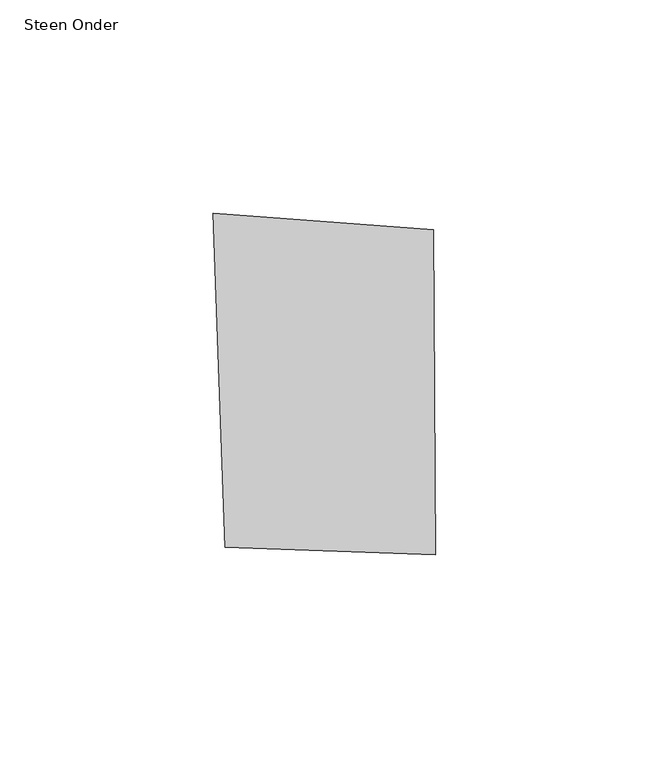
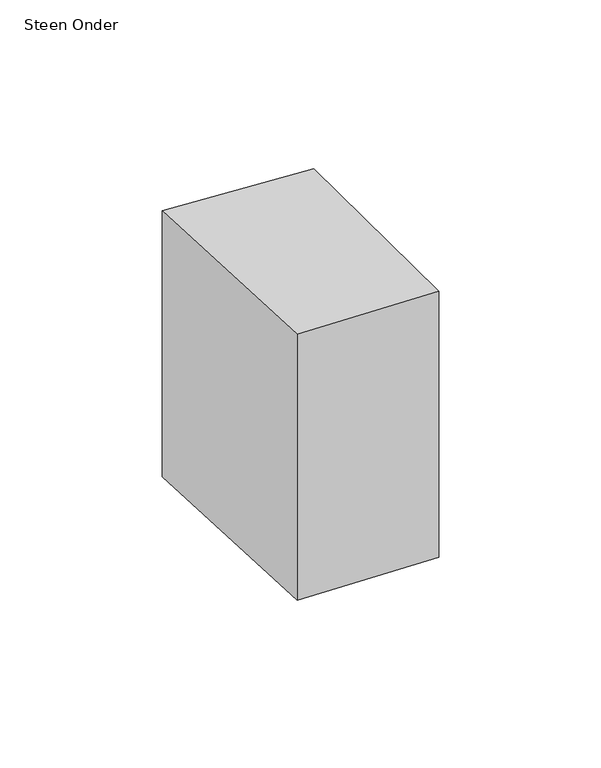
"""IFC4 building model written with IfcOpenShell, lengths in millimetres: proxy geometry, 00_GMA_steen_versie_4 : Steen Onder."""

from ifc_helpers import new_model, si_unit, origin, origin_with_axes, place, context, project, spatial, polyline, outline, extrude, source, transform, mapped, element, save


def steen_onder_7befe764(model_context):
    return source(origin(), model_context, "Body", "SweptSolid", [
        extrude(outline(polyline([(100.3327975, 104.5668366), (100.8339112, 28.4196095), (51.568424, 30.0955228), (48.7496867, 108.3562833), (100.3327975, 104.5668366)])), origin_with_axes(), (0.0, 0.0, 1.0), 100.0),
    ])


if __name__ == "__main__":
    model = new_model("IFC4")
    model_context = context("Model", 3, world=origin())
    ifc_project = project(units=[si_unit("LENGTHUNIT", "METRE", prefix="MILLI")], contexts=[model_context])
    site = spatial("IfcSite", under=ifc_project)
    building = spatial("IfcBuilding", under=site)
    placement = place(None, origin())
    steen_onder_shape = steen_onder_7befe764(model_context)
    element("IfcBuildingElementProxy", 1, Name="00_GMA_steen_versie_4 : Steen Onder", ObjectType="00_GMA_steen_versie_4 : Steen Onder", at=placement, inside=building, context=model_context, shape_type="MappedRepresentation", body=[
        mapped(steen_onder_shape, transform((0.0, 0.0, 0.0), x_axis=(1.0, 0.0, 0.0), y_axis=(0.0, 1.0, 0.0), z_axis=(0.0, 0.0, 1.0))),
    ])
    save(model, "model.ifc")

# Revit data of these elements
# Type "00_GMA_steen_versie_4 : Steen Onder"
#   StootVoegHalfBoven [instance default] = 5 mm
#   StootVoegHalf [instance default] = 5 mm
#   StootVoegBreedteOnder = 10 mm
#   StootVoegBreedteBoven = 10 mm
#   Steendikte = 100 mm
#   LintVoegOnderHalf = 0 mm
#   LintVoegOnder = 0 mm
#   LintVoegBovenHalf = 5 mm
#   LintVoegBoven = 10 mm
#   materiaal = none
#   MateriaalVoeg = none
#   Default Elevation = 0
